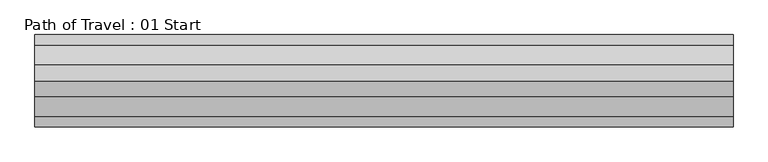
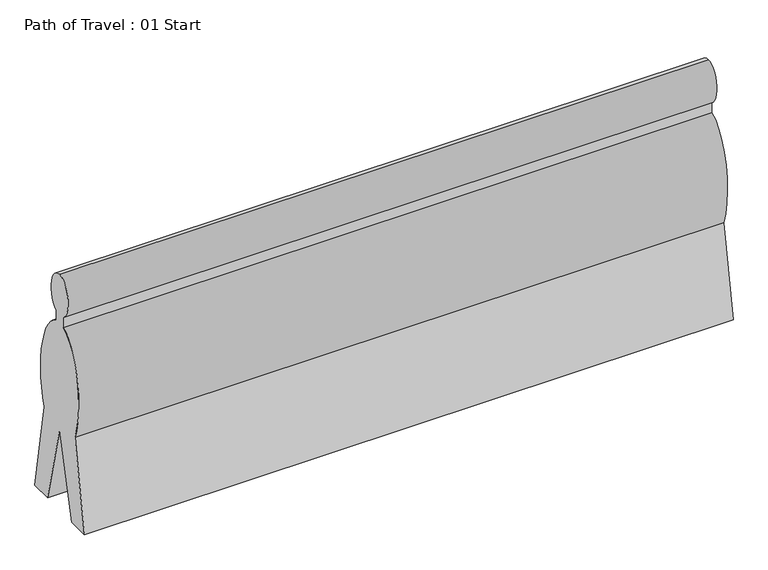
"""IFC4 building model written with IfcOpenShell, lengths in millimetres: proxy geometry, Path of Travel : 01 Start."""

from ifc_helpers import new_model, si_unit, point, frame, origin, place, context, project, spatial, ellipse_curve, trimmed, source, transform, mapped, element, save
from ifc_brep_helpers import plane_surface, extruded_surface, advanced_brep


def path_of_travel_01_start_02bedfe9(model_context):
    return source(origin(), model_context, "Body", "AdvancedBrep", [
        advanced_brep(
        [(227.5554837, 0.0, 1727.2), (227.5554837, 42.9018657, 1436.6534209), (227.5554837, 42.9018657, 1363.4763406), (227.5554837, 184.1186263, 643.4144547), (227.5554837, 297.5699544, 0.0), (227.5554837, 145.6574193, 0.0), (227.5554837, 0.0, 584.2), (227.5554837, -145.6574193, 0.0), (227.5554837, -297.5699544, 0.0), (227.5554837, -184.1186263, 643.4144547), (227.5554837, -42.9018657, 1363.4763406), (227.5554837, -42.9018657, 1436.6534209), (4723.3554837, 0.0, 1727.2), (4723.3554837, -42.9018657, 1436.6534209), (4723.3554837, -42.9018657, 1363.4763406), (4723.3554837, -184.1186263, 643.4144547), (4723.3554837, -297.5699544, 0.0), (4723.3554837, -145.6574193, 0.0), (4723.3554837, 0.0, 584.2), (4723.3554837, 145.6574193, 0.0), (4723.3554837, 297.5699544, 0.0), (4723.3554837, 184.1186263, 643.4144547), (4723.3554837, 42.9018657, 1363.4763406), (4723.3554837, 42.9018657, 1436.6534209)],
        [
            (0, 1, ellipse_curve(frame((227.5554837, 0.0, 1574.8), z_axis=(-1.0, 0.0, 0.0), x_axis=(0.0, 0.0, 1.0)), 152.4, 101.6)),
            (1, 2),
            (2, 3, ellipse_curve(frame((227.5554837, 0.0, 914.4), z_axis=(-1.0, 0.0, 0.0), x_axis=(0.0, 0.0, -1.0)), 457.2, 228.6)),
            (3, 4),
            (4, 5),
            (5, 6),
            (6, 7),
            (7, 8),
            (8, 9),
            (9, 10, ellipse_curve(frame((227.5554837, 0.0, 914.4), z_axis=(-1.0, 0.0, 0.0), x_axis=(0.0, 0.0, -1.0)), 457.2, 228.6)),
            (10, 11),
            (11, 0, ellipse_curve(frame((227.5554837, 0.0, 1574.8), z_axis=(-1.0, 0.0, 0.0), x_axis=(0.0, 0.0, 1.0)), 152.4, 101.6)),
            (12, 13, ellipse_curve(frame((4723.3554837, 0.0, 1574.8), z_axis=(1.0, 0.0, 0.0), x_axis=(0.0, 0.0, 1.0)), 152.4, 101.6)),
            (13, 14),
            (14, 15, ellipse_curve(frame((4723.3554837, 0.0, 914.4), z_axis=(1.0, 0.0, 0.0), x_axis=(0.0, 0.0, -1.0)), 457.2, 228.6)),
            (15, 16),
            (16, 17),
            (17, 18),
            (18, 19),
            (19, 20),
            (20, 21),
            (21, 22, ellipse_curve(frame((4723.3554837, 0.0, 914.4), z_axis=(1.0, 0.0, 0.0), x_axis=(0.0, 0.0, -1.0)), 457.2, 228.6)),
            (22, 23),
            (23, 12, ellipse_curve(frame((4723.3554837, 0.0, 1574.8), z_axis=(1.0, 0.0, 0.0), x_axis=(0.0, 0.0, 1.0)), 152.4, 101.6)),
            (0, 12),
            (23, 1),
            (22, 2),
            (21, 3),
            (20, 4),
            (19, 5),
            (18, 6),
            (17, 7),
            (16, 8),
            (15, 9),
            (14, 10),
            (13, 11),
        ],
        [
            plane_surface(frame((227.5554837, 0.0, 0.0), z_axis=(-1.0, 0.0, 0.0), x_axis=(0.0, 0.0, 1.0))),
            plane_surface(frame((4723.3554837, 0.0, 0.0), z_axis=(1.0, 0.0, 0.0), x_axis=(0.0, 0.0, 1.0))),
            extruded_surface(trimmed(ellipse_curve(frame((4723.3554837, 0.0, 1574.8), z_axis=(-1.0, 0.0, 0.0), x_axis=(0.0, 0.0, 1.0)), 152.4, 101.6), [point((4723.3554837, 0.0, 1727.2))], [point((4723.3554837, 42.9018657, 1436.6534209))], True, "CARTESIAN"), (-4495.8, 0.0, 0.0), 4495.8),
            plane_surface(frame((227.5554837, 42.9018657, 1436.6534209), z_axis=(0.0, 1.0, 0.0), x_axis=(1.0, 0.0, 0.0))),
            extruded_surface(trimmed(ellipse_curve(frame((4723.3554837, 0.0, 914.4), z_axis=(-1.0, 0.0, 0.0), x_axis=(0.0, 0.0, -1.0)), 457.2, 228.6), [point((4723.3554837, 42.9018657, 1363.4763406))], [point((4723.3554837, 184.1186263, 643.4144547))], True, "CARTESIAN"), (-4495.8, 0.0, 0.0), 4495.8),
            plane_surface(frame((227.5554837, 184.1186263, 643.4144547), z_axis=(0.0, 0.9848077530122078, 0.17364817766693205), x_axis=(1.0, 0.0, 0.0))),
            plane_surface(frame((227.5554837, 297.5699544, 0.0), z_axis=(0.0, 0.0, -1.0), x_axis=(1.0, 0.0, 0.0))),
            plane_surface(frame((227.5554837, 145.6574193, 0.0), z_axis=(0.0, -0.9702957262760199, -0.2419218955995739), x_axis=(1.0, 0.0, 0.0))),
            plane_surface(frame((227.5554837, 0.0, 584.2), z_axis=(0.0, 0.9702957262759961, -0.24192189559966923), x_axis=(1.0, 0.0, 0.0))),
            plane_surface(frame((227.5554837, -145.6574193, 0.0), z_axis=(0.0, 0.0, -1.0), x_axis=(1.0, 0.0, 0.0))),
            plane_surface(frame((227.5554837, -297.5699544, 0.0), z_axis=(0.0, -0.984807753012208, 0.17364817766693066), x_axis=(1.0, 0.0, 0.0))),
            extruded_surface(trimmed(ellipse_curve(frame((4723.3554837, 0.0, 914.4), z_axis=(-1.0, 0.0, 0.0), x_axis=(0.0, 0.0, -1.0)), 457.2, 228.6), [point((4723.3554837, -184.1186263, 643.4144547))], [point((4723.3554837, -42.9018657, 1363.4763406))], True, "CARTESIAN"), (-4495.8, 0.0, 0.0), 4495.8),
            plane_surface(frame((227.5554837, -42.9018657, 1363.4763406), z_axis=(0.0, -1.0, 0.0), x_axis=(1.0, 0.0, 0.0))),
            extruded_surface(trimmed(ellipse_curve(frame((4723.3554837, 0.0, 1574.8), z_axis=(-1.0, 0.0, 0.0), x_axis=(0.0, 0.0, 1.0)), 152.4, 101.6), [point((4723.3554837, -42.9018657, 1436.6534209))], [point((4723.3554837, 0.0, 1727.2))], True, "CARTESIAN"), (-4495.8, 0.0, 0.0), 4495.8),
        ],
        [
            (0, [[1, 2, 3, 4, 5, 6, 7, 8, 9, 10, 11, 12]]),
            (1, [[13, 14, 15, 16, 17, 18, 19, 20, 21, 22, 23, 24]]),
            (2, [[-1, 25, -24, 26]]),
            (3, [[-2, -26, -23, 27]]),
            (4, [[-3, -27, -22, 28]]),
            (5, [[-4, -28, -21, 29]]),
            (6, [[-5, -29, -20, 30]]),
            (7, [[-6, -30, -19, 31]]),
            (8, [[-7, -31, -18, 32]]),
            (9, [[-8, -32, -17, 33]]),
            (10, [[-9, -33, -16, 34]]),
            (11, [[-10, -34, -15, 35]]),
            (12, [[-11, -35, -14, 36]]),
            (13, [[-12, -36, -13, -25]]),
        ],
    ),
    ])


if __name__ == "__main__":
    model = new_model("IFC4")
    model_context = context("Model", 3, world=origin())
    ifc_project = project(units=[si_unit("LENGTHUNIT", "METRE", prefix="MILLI")], contexts=[model_context])
    site = spatial("IfcSite", under=ifc_project)
    building = spatial("IfcBuilding", under=site)
    placement = place(None, origin())
    path_of_travel_01_start_shape = path_of_travel_01_start_02bedfe9(model_context)
    element("IfcBuildingElementProxy", 1, Name="Path of Travel : 01 Start", ObjectType="Path of Travel : 01 Start", at=placement, inside=building, context=model_context, shape_type="MappedRepresentation", body=[
        mapped(path_of_travel_01_start_shape, transform((0.0, 0.0, 0.0), x_axis=(1.0, 0.0, 0.0), y_axis=(0.0, 1.0, 0.0), z_axis=(0.0, 0.0, 1.0))),
    ])
    save(model, "model.ifc")

# Revit data of these elements
# Type "Path of Travel : 01 Start"
#   Path of Egress [instance default] = 4' - 0"
#   built-in parameter 1001306 [instance default] = 4 (stored number, unit not read)
#   Dot at Start = yes
#   Arrow in Middle = yes
#   Arrow at End = no
#   Egress Path = none
# Element 1 (IfcBuildingElementProxy, "Path of Travel : 01 Start")
#   Path of Egress = 14' - 9"
#   built-in parameter 1001306 = 14.75 (stored number, unit not read)
#   Materials on its faces: "Egress Path Solid"
# Materials
#   "Egress Path Solid": class "Unassigned", colour RGB 255 128 64, transparency 0.75, Comments = "Rendering appearance not upgraded "
